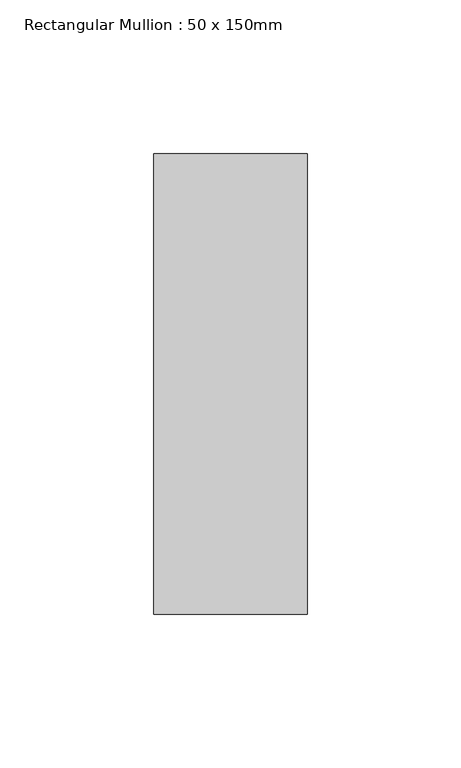
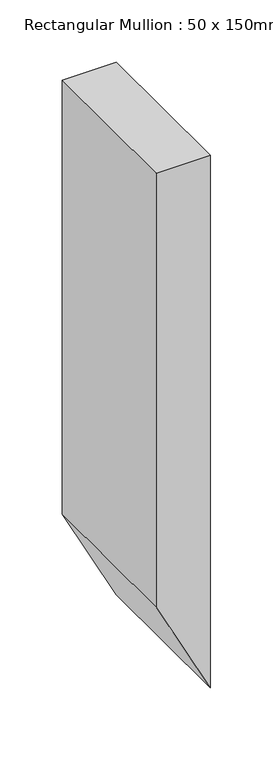
"""IFC4 building model written with IfcOpenShell, lengths in millimetres: member geometry, Rectangular Mullion : 50 x 150mm."""

from ifc_helpers import new_model, si_unit, frame, origin, place, context, project, spatial, polyline, outline, extrude, source, transform, mapped, element, save


def rectangular_mullion_50_x_150mm_25409b62(model_context):
    return source(origin(), model_context, "Body", "SweptSolid", [
        extrude(outline(polyline([(0.0, 0.0), (0.0, -50.0), (-424.2829548, -50.0), (-520.3320611, 0.0), (0.0, 0.0)])), frame((0.0, -75.0, 0.0), z_axis=(0.0, 1.0, 0.0), x_axis=(0.0, 0.0, 1.0)), (0.0, 0.0, 1.0), 150.0),
    ])


if __name__ == "__main__":
    model = new_model("IFC4")
    model_context = context("Model", 3, world=origin())
    ifc_project = project(units=[si_unit("LENGTHUNIT", "METRE", prefix="MILLI")], contexts=[model_context])
    site = spatial("IfcSite", under=ifc_project)
    building = spatial("IfcBuilding", under=site)
    placement = place(None, origin())
    rectangular_mullion_50_x_150mm_shape = rectangular_mullion_50_x_150mm_25409b62(model_context)
    element("IfcMember", 1, ObjectType="Rectangular Mullion : 50 x 150mm", at=placement, inside=building, context=model_context, shape_type="MappedRepresentation", body=[
        mapped(rectangular_mullion_50_x_150mm_shape, transform((0.0, 0.0, 0.0), x_axis=(1.0, 0.0, 0.0), y_axis=(0.0, 1.0, 0.0), z_axis=(0.0, 0.0, 1.0))),
    ])
    save(model, "model.ifc")

# Revit data of these elements
# Type "Rectangular Mullion : 50 x 150mm"
#   built-in parameter 1007304 = 0.492126 (stored number, unit not read)
#   built-in parameter 1007301 = 0.082021 (stored number, unit not read)
#   built-in parameter 1007300 = 0.082021 (stored number, unit not read)
# Element 1 (IfcMember, "Rectangular Mullion : 50 x 150mm")
#   Materials on its faces: "Aluminium"
# Materials
#   "Aluminium": class "Metal", colour RGB 247 247 247, transparency 0, Description = "Aluminium 6061", Cost = 0
